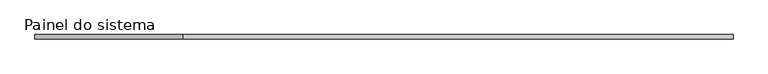
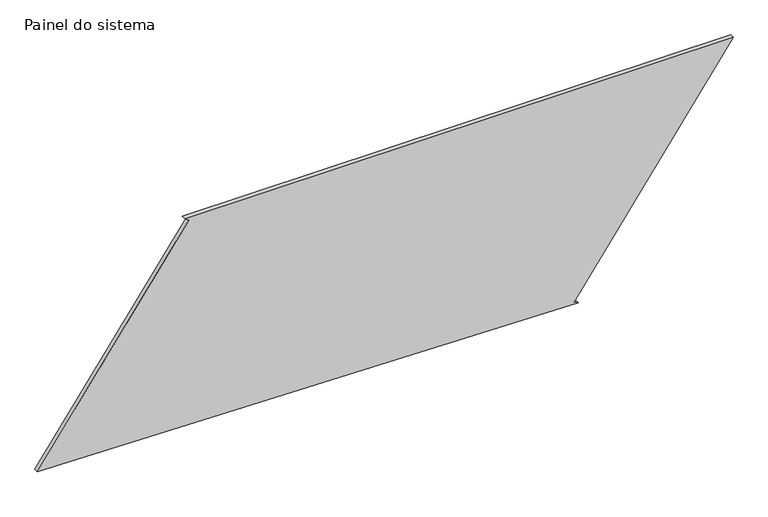
"""IFC4 building model written with IfcOpenShell, lengths in millimetres: plate geometry, Painel do sistema : Envidraçado."""

from ifc_helpers import new_model, si_unit, frame, origin, place, context, project, spatial, polyline, outline, extrude, source, transform, mapped, element, save


def painel_do_sistema_5004c774(model_context):
    return source(origin(), model_context, "Body", "SweptSolid", [
        extrude(outline(polyline([(0.0, 1098.2821493), (14.4529738, 1077.8833369), (1289.7205911, 1981.4364014), (1289.7205911, -1140.8396482), (1275.2676173, -1120.4408357), (60.0653158, -1981.4364014), (0.0, 1098.2821493)])), frame((0.0, 24.5, 0.0), z_axis=(0.0, 1.0, 0.0), x_axis=(0.0, 0.0, 1.0)), (0.0, 0.0, 1.0), 25.0),
    ])


if __name__ == "__main__":
    model = new_model("IFC4")
    model_context = context("Model", 3, world=origin())
    ifc_project = project(units=[si_unit("LENGTHUNIT", "METRE", prefix="MILLI")], contexts=[model_context])
    site = spatial("IfcSite", under=ifc_project)
    building = spatial("IfcBuilding", under=site)
    placement = place(None, origin())
    painel_do_sistema_shape = painel_do_sistema_5004c774(model_context)
    element("IfcPlate", 1, ObjectType="Painel do sistema : Envidraçado", at=placement, inside=building, context=model_context, shape_type="MappedRepresentation", body=[
        mapped(painel_do_sistema_shape, transform((0.0, 0.0, 0.0), x_axis=(1.0, 0.0, 0.0), y_axis=(0.0, 1.0, 0.0), z_axis=(0.0, 0.0, 1.0))),
    ])
    save(model, "model.ifc")

# Revit data of these elements
# Type "Painel do sistema : Envidraçado"
#   Construction Type Id = "GSP4R"
#   Analytic Construction = "Vidraça única Pilkington 1/8 pol"
#   Visual Light Transmittance = 0.9
#   Solar Heat Gain Coefficient = 0.86
#   Heat Transfer Coefficient (U) = 6.7069 W/(m²·K)
# Element 1 (IfcPlate, "Painel do sistema : Envidraçado")
#   Materials on its faces: "Vidro"
# Materials
#   "Vidro": class "Vidro", colour RGB 0 128 192, transparency 0.9, Description = "Vidro de sílica", Cost = 0
